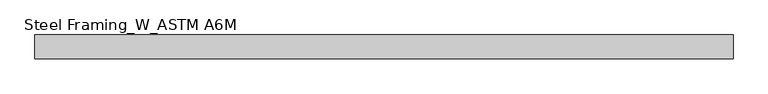
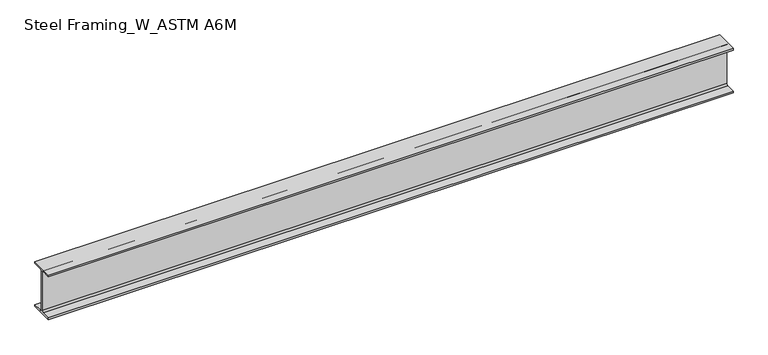
"""IFC4 building model written with IfcOpenShell, lengths in millimetres: beam geometry, Steel Framing_W_ASTM A6M : H_SB_AR_S02_W200x22.5_RB5."""

from ifc_helpers import new_model, si_unit, point, frame, frame_2d, origin, place, context, project, spatial, polyline, circle_curve, trimmed, segment, composite_curve, outline, extrude, source, transform, mapped, element, save


def steel_framing_w_astm_a6m_49e40538(model_context):
    return source(origin(), model_context, "Body", "SweptSolid", [
        extrude(outline(composite_curve([segment(polyline([(51.0, -95.0), (51.0, -103.0), (-51.0, -103.0), (-51.0, -95.0), (-10.71, -95.0)]), True, "CONTINUOUS"), segment(trimmed(circle_curve(frame_2d((-10.71, -87.4)), 7.6), [point((-10.71, -95.0))], [point((-3.11, -87.4))], True, "CARTESIAN"), True, "CONTINUOUS"), segment(polyline([(-3.11, -87.4), (-3.11, 87.4)]), True, "CONTINUOUS"), segment(trimmed(circle_curve(frame_2d((-10.71, 87.4)), 7.6), [point((-3.11, 87.4))], [point((-10.71, 95.0))], True, "CARTESIAN"), True, "CONTINUOUS"), segment(polyline([(-10.71, 95.0), (-51.0, 95.0), (-51.0, 103.0), (51.0, 103.0), (51.0, 95.0), (10.71, 95.0)]), True, "CONTINUOUS"), segment(trimmed(circle_curve(frame_2d((10.71, 87.4)), 7.6), [point((10.71, 95.0))], [point((3.11, 87.4))], True, "CARTESIAN"), True, "CONTINUOUS"), segment(polyline([(3.11, 87.4), (3.11, -87.4)]), True, "CONTINUOUS"), segment(trimmed(circle_curve(frame_2d((10.71, -87.4)), 7.6), [point((3.11, -87.4))], [point((10.71, -95.0))], True, "CARTESIAN"), True, "CONTINUOUS"), segment(polyline([(10.71, -95.0), (51.0, -95.0)]), True, "CONTINUOUS")], self_intersect=False)), frame((-1500.0, 0.0, 0.0), z_axis=(1.0, 0.0, 0.0), x_axis=(0.0, 1.0, 0.0)), (0.0, 0.0, 1.0), 2987.2),
    ])


if __name__ == "__main__":
    model = new_model("IFC4")
    model_context = context("Model", 3, world=origin())
    ifc_project = project(units=[si_unit("LENGTHUNIT", "METRE", prefix="MILLI")], contexts=[model_context])
    site = spatial("IfcSite", under=ifc_project)
    building = spatial("IfcBuilding", under=site)
    placement = place(None, origin())
    steel_framing_w_astm_a6m_shape = steel_framing_w_astm_a6m_49e40538(model_context)
    element("IfcBeam", 1, ObjectType="Steel Framing_W_ASTM A6M : H_SB_AR_S02_W200x22.5_RB5", at=placement, inside=building, context=model_context, shape_type="MappedRepresentation", body=[
        mapped(steel_framing_w_astm_a6m_shape, transform((0.0, 0.0, 0.0), x_axis=(1.0, 0.0, 0.0), y_axis=(0.0, 1.0, 0.0), z_axis=(0.0, 0.0, 1.0))),
    ])
    save(model, "model.ifc")

# Revit data of these elements
# Type "Steel Framing_W_ASTM A6M : H_SB_AR_S02_W200x22.5_RB5"
#   Type Mark = "RB5"
#   Section Name Key = "W8x15"
#   Width = 10.2 cm
#   Web Thickness = 0.622 cm
#   Web Fillet = 0.76 cm
#   Warping Constant = 13900.0 cm⁶
#   Torsional Moment of Inertia = 5.70 cm⁴
#   Section Area = 28.6 cm²
#   Plastic Modulus weak axis = 43.8 cm³
#   Plastic Modulus strong axis = 223.0 cm³
#   Perimeter = 0.795 m²/m
#   Nominal Weight = 22.50 kgf/m
#   Moment of Inertia weak axis = 142.00 cm⁴
#   Moment of Inertia strong axis = 2000.00 cm⁴
#   Height = 20.6 cm
#   Flange Thickness = 0.8 cm
#   Elastic Modulus weak axis = 27.9 cm³
#   Elastic Modulus strong axis = 193.0 cm³
#   Centroid Vertical = 10.3 cm
#   Centroid Horizontal = 5.1 cm
#   Length [instance default] = 1500 mm
#   Structural Material [instance default] = Steel, 45-345
#   Bolt Spacing = 0
#   Assembly Code = ""
# Element 1 (IfcBeam, "Steel Framing_W_ASTM A6M : H_SB_AR_S02_W200x22.5_RB5")
#   Materials on its faces: "Steel, 45-345"
# Materials
#   "Steel, 45-345": class "Metal", colour RGB 189 187 185, transparency 0, Description = "Steel 345 MPa", Cost = 0
